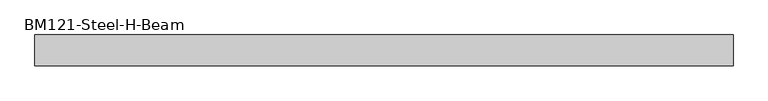
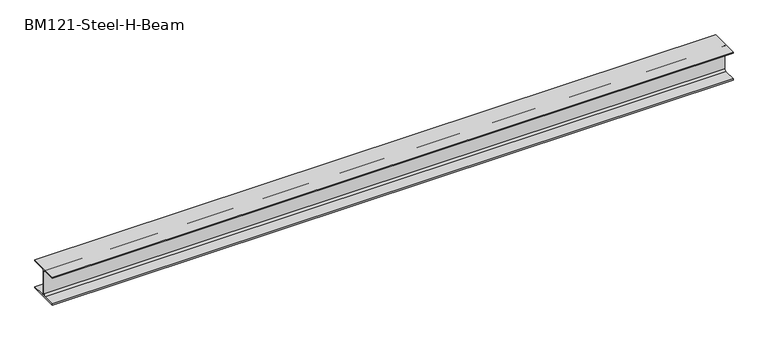
"""IFC4 building model written with IfcOpenShell, lengths in millimetres: beam geometry, BM121-Steel-H-Beam : BM121_H-294×302x12x12."""

from ifc_helpers import new_model, si_unit, point, frame, frame_2d, origin, place, context, project, spatial, polyline, circle_curve, trimmed, segment, composite_curve, outline, extrude, source, transform, mapped, element, save


def bm121_steel_h_beam_5c21d0b8(model_context):
    return source(origin(), model_context, "Body", "SweptSolid", [
        extrude(outline(composite_curve([segment(polyline([(-151.0, 147.0), (151.0, 147.0), (151.0, 135.0), (24.0, 135.0)]), True, "CONTINUOUS"), segment(trimmed(circle_curve(frame_2d((24.0, 117.0)), 18.0), [point((24.0, 135.0))], [point((6.0, 117.0))], True, "CARTESIAN"), True, "CONTINUOUS"), segment(polyline([(6.0, 117.0), (6.0, -117.0)]), True, "CONTINUOUS"), segment(trimmed(circle_curve(frame_2d((24.0, -117.0)), 18.0), [point((6.0, -117.0))], [point((24.0, -135.0))], True, "CARTESIAN"), True, "CONTINUOUS"), segment(polyline([(24.0, -135.0), (151.0, -135.0), (151.0, -147.0), (-151.0, -147.0), (-151.0, -135.0), (-24.0, -135.0)]), True, "CONTINUOUS"), segment(trimmed(circle_curve(frame_2d((-24.0, -117.0)), 18.0), [point((-24.0, -135.0))], [point((-6.0, -117.0))], True, "CARTESIAN"), True, "CONTINUOUS"), segment(polyline([(-6.0, -117.0), (-6.0, 117.0)]), True, "CONTINUOUS"), segment(trimmed(circle_curve(frame_2d((-24.0, 117.0)), 18.0), [point((-6.0, 117.0))], [point((-24.0, 135.0))], True, "CARTESIAN"), True, "CONTINUOUS"), segment(polyline([(-24.0, 135.0), (-151.0, 135.0), (-151.0, 147.0)]), True, "CONTINUOUS")], self_intersect=False)), frame((-3401.1, 0.0, 0.0), z_axis=(1.0, 0.0, 0.0), x_axis=(0.0, 1.0, 0.0)), (0.0, 0.0, 1.0), 6802.2),
    ])


if __name__ == "__main__":
    model = new_model("IFC4")
    model_context = context("Model", 3, world=origin())
    ifc_project = project(units=[si_unit("LENGTHUNIT", "METRE", prefix="MILLI")], contexts=[model_context])
    site = spatial("IfcSite", under=ifc_project)
    building = spatial("IfcBuilding", under=site)
    placement = place(None, origin())
    bm121_steel_h_beam_shape = bm121_steel_h_beam_5c21d0b8(model_context)
    element("IfcBeam", 1, ObjectType="BM121-Steel-H-Beam : BM121_H-294×302x12x12", at=placement, inside=building, context=model_context, shape_type="MappedRepresentation", body=[
        mapped(bm121_steel_h_beam_shape, transform((0.0, 0.0, 0.0), x_axis=(1.0, 0.0, 0.0), y_axis=(0.0, 1.0, 0.0), z_axis=(0.0, 0.0, 1.0))),
    ])
    save(model, "model.ifc")

# Revit data of these elements
# Type "BM121-Steel-H-Beam : BM121_H-294×302x12x12"
#   tw = 12 mm
#   tf = 12 mm
#   r = 18 mm
#   bf = 302 mm
#   Unit Weight = 84.50 kg/m
#   Surface Area = 1.7411 m²/m
#   Length [instance default] = 3000 mm
#   H = 294 mm
#   Sectional Area = 10770.0 cm²
